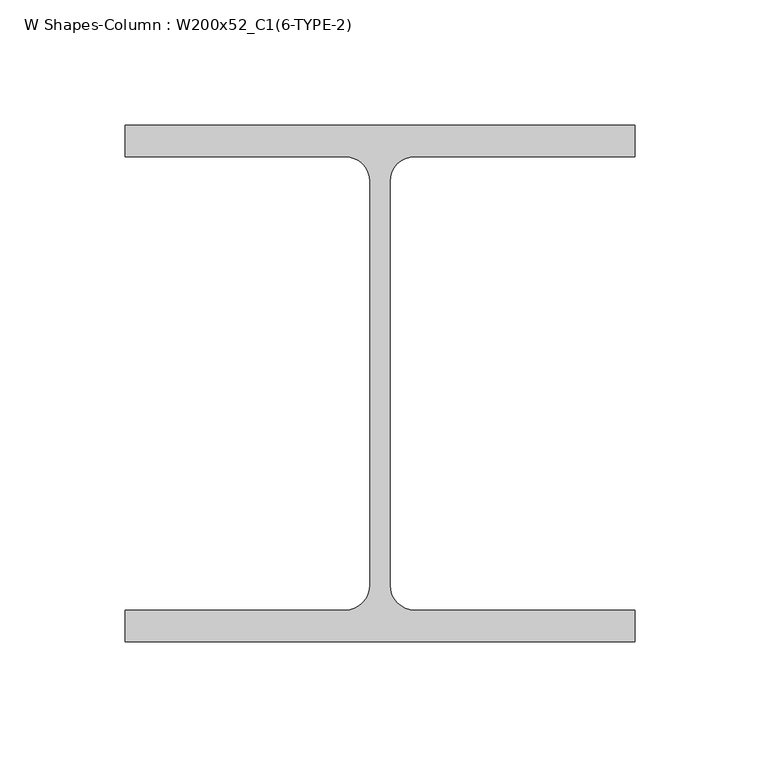
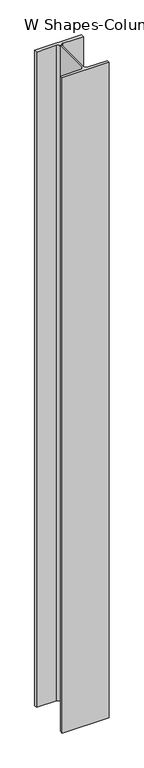
"""IFC4 building model written with IfcOpenShell, lengths in millimetres: column geometry, W Shapes-Column : W200x52_C1(6-TYPE-2)."""

from ifc_helpers import new_model, si_unit, point, frame, frame_2d, origin, place, context, project, spatial, polyline, circle_curve, trimmed, segment, composite_curve, outline, extrude, source, transform, mapped, element, save


def w_shapes_column_w200x52_c1_6_type_2_39bb5361(model_context):
    return source(origin(), model_context, "Body", "SweptSolid", [
        extrude(outline(composite_curve([segment(polyline([(101.854, 103.124), (101.854, 90.551), (13.9446, 90.551)]), True, "CONTINUOUS"), segment(trimmed(circle_curve(frame_2d((13.9446, 80.5434)), 10.0076), [point((13.9446, 90.551))], [point((3.937, 80.5434))], True, "CARTESIAN"), True, "CONTINUOUS"), segment(polyline([(3.937, 80.5434), (3.937, -80.5434)]), True, "CONTINUOUS"), segment(trimmed(circle_curve(frame_2d((13.9446, -80.5434)), 10.0076), [point((3.937, -80.5434))], [point((13.9446, -90.551))], True, "CARTESIAN"), True, "CONTINUOUS"), segment(polyline([(13.9446, -90.551), (101.854, -90.551), (101.854, -103.124), (-101.854, -103.124), (-101.854, -90.551), (-13.9446, -90.551)]), True, "CONTINUOUS"), segment(trimmed(circle_curve(frame_2d((-13.9446, -80.5434)), 10.0076), [point((-13.9446, -90.551))], [point((-3.937, -80.5434))], True, "CARTESIAN"), True, "CONTINUOUS"), segment(polyline([(-3.937, -80.5434), (-3.937, 80.5434)]), True, "CONTINUOUS"), segment(trimmed(circle_curve(frame_2d((-13.9446, 80.5434)), 10.0076), [point((-3.937, 80.5434))], [point((-13.9446, 90.551))], True, "CARTESIAN"), True, "CONTINUOUS"), segment(polyline([(-13.9446, 90.551), (-101.854, 90.551), (-101.854, 103.124), (101.854, 103.124)]), True, "CONTINUOUS")], self_intersect=False)), frame((0.0, 0.0, 9760.0), z_axis=(0.0, 0.0, 1.0), x_axis=(1.0, 0.0, 0.0)), (0.0, 0.0, 1.0), 3000.0),
    ])


if __name__ == "__main__":
    model = new_model("IFC4")
    model_context = context("Model", 3, world=origin())
    ifc_project = project(units=[si_unit("LENGTHUNIT", "METRE", prefix="MILLI")], contexts=[model_context])
    site = spatial("IfcSite", under=ifc_project)
    building = spatial("IfcBuilding", under=site)
    placement = place(None, origin())
    w_shapes_column_w200x52_c1_6_type_2_shape = w_shapes_column_w200x52_c1_6_type_2_39bb5361(model_context)
    element("IfcColumn", 1, ObjectType="W Shapes-Column : W200x52_C1(6-TYPE-2)", at=placement, inside=building, context=model_context, shape_type="MappedRepresentation", body=[
        mapped(w_shapes_column_w200x52_c1_6_type_2_shape, transform((0.0, 0.0, 0.0), x_axis=(1.0, 0.0, 0.0), y_axis=(0.0, 1.0, 0.0), z_axis=(0.0, 0.0, 1.0))),
    ])
    save(model, "model.ifc")

# Revit data of these elements
# Type "W Shapes-Column : W200x52_C1(6-TYPE-2)"
#   Section Name Key = "W8X35"
#   Assembly Code = "B10"
#   Width = 20.3708 cm
#   Web Thickness = 0.7874 cm
#   Web Fillet = 1.0008 cm
#   Warping Constant = 166223.7 cm⁶
#   Torsional Moment of Inertia = 32.0082 cm⁴
#   Section Area = 66.4515 cm²
#   Plastic Modulus weak axis = 263.832 cm³
#   Plastic Modulus strong axis = 568.631 cm³
#   Perimeter = 1.1936 m²/m
#   Nominal Weight = 52.0857 kgf/m
#   Moment of Inertia weak axis = 1773.15 cm⁴
#   Moment of Inertia strong axis = 5286.14 cm⁴
#   Height = 20.6248 cm
#   Flange Thickness = 1.2573 cm
#   Elastic Modulus weak axis = 173.703 cm³
#   Elastic Modulus strong axis = 511.276 cm³
#   Clear Web Height = 14.605 cm
#   Centroid Vertical = 10.3124 cm
#   Centroid Horizontal = 10.1854 cm
#   Bolt Spacing = 13.97 cm
#   Structural Material [instance default] = Steel ASTM A992
#   Principal Axes Angle = 0
# Element 1 (IfcColumn, "W Shapes-Column : W200x52_C1(6-TYPE-2)")
#   Structural Material = none
# Materials
#   "Steel ASTM A992": class "Metal", colour RGB 199 199 199, transparency 0, Description = "Structural steel 50ksi", Cost = 0
